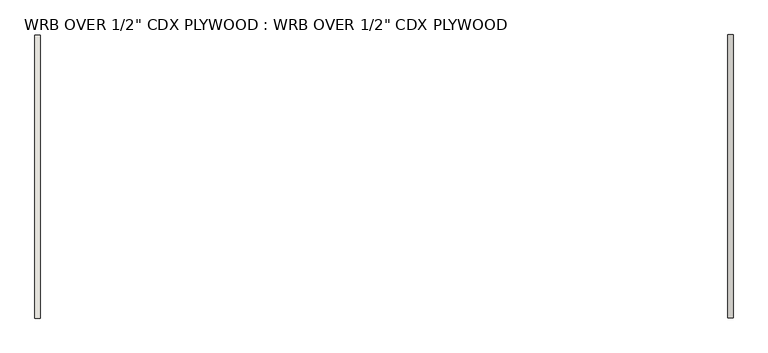
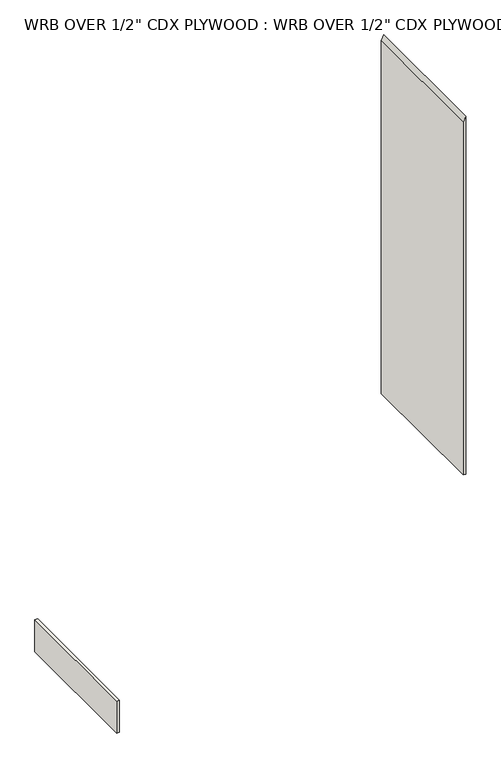
"""IFC4 building model written with IfcOpenShell, lengths in millimetres: wall geometry."""

from ifc_helpers import new_model, si_unit, frame, origin, place, context, project, spatial, polyline, outline, extrude, source, transform, mapped, element, save


def wall_4e3e3ca6(model_context):
    return source(origin(), model_context, "Body", "SweptSolid", [
        extrude(outline(polyline([(17933.1870052, -2319.6634634), (17920.4870052, -2319.6634634), (17920.4870052, -1633.8634634), (17933.1870052, -1633.8634634), (17933.1870052, -2319.6634634)])), frame((0.0, 0.0, 2197.1), z_axis=(0.0, 0.0, 1.0), x_axis=(1.0, 0.0, 0.0)), (0.0, 0.0, 1.0), 164.2249455),
        extrude(outline(polyline([(4737.4557155, 19596.8870052), (2931.649464, 19596.8870052), (2931.649464, 19609.5870052), (4762.8557155, 19609.5870052), (4737.4557155, 19596.8870052)])), frame((0.0, -2319.6634634, 0.0), z_axis=(0.0, 1.0, 0.0), x_axis=(0.0, 0.0, 1.0)), (0.0, 0.0, 1.0), 685.8),
    ])


if __name__ == "__main__":
    model = new_model("IFC4")
    model_context = context("Model", 3, world=origin())
    ifc_project = project(units=[si_unit("LENGTHUNIT", "METRE", prefix="MILLI")], contexts=[model_context])
    site = spatial("IfcSite", under=ifc_project)
    building = spatial("IfcBuilding", under=site)
    placement = place(None, origin())
    wall_shape = wall_4e3e3ca6(model_context)
    element("IfcWall", 1, ObjectType="WRB OVER 1/2\" CDX PLYWOOD : WRB OVER 1/2\" CDX PLYWOOD", at=placement, inside=building, context=model_context, shape_type="MappedRepresentation", body=[
        mapped(wall_shape, transform((0.0, 0.0, 0.0), x_axis=(1.0, 0.0, 0.0), y_axis=(0.0, 1.0, 0.0), z_axis=(0.0, 0.0, 1.0))),
    ])
    save(model, "model.ifc")

# Revit data of these elements
# Element 1 (IfcWall, "WRB OVER 1/2\" CDX PLYWOOD : WRB OVER 1/2\" CDX PLYWOOD")
#   Materials on its faces: "WRB OVER 1\" STRUCTURAL INSULATED SHEATHING (R-3.6)"
# Materials
#   "WRB OVER 1\" STRUCTURAL INSULATED SHEATHING (R-3.6)": class "Unassigned", colour RGB 196 177 123, transparency 0, Cost = 0
